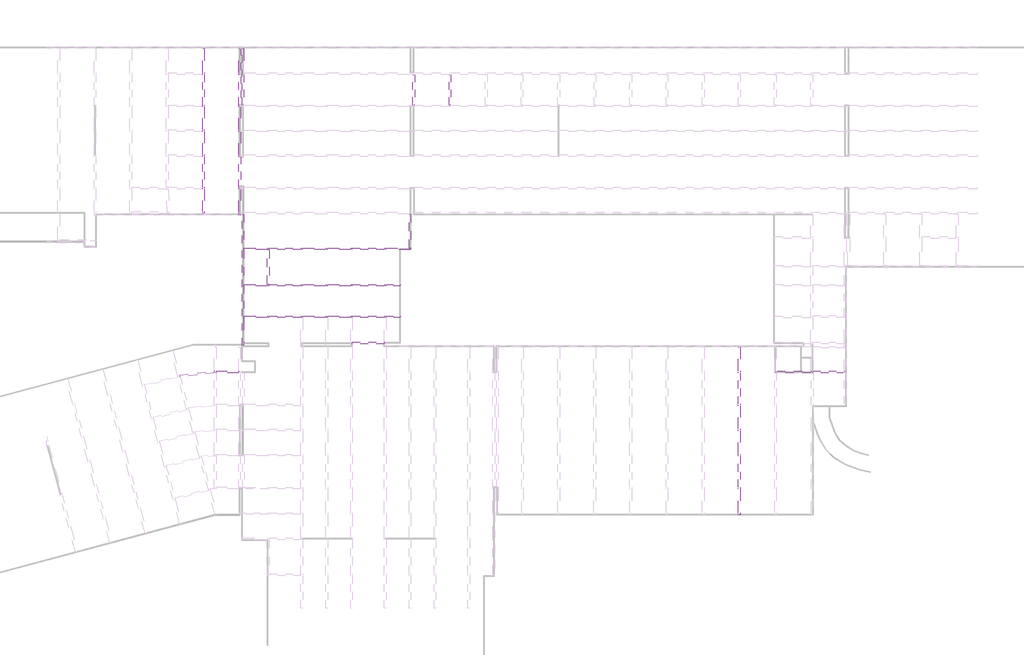
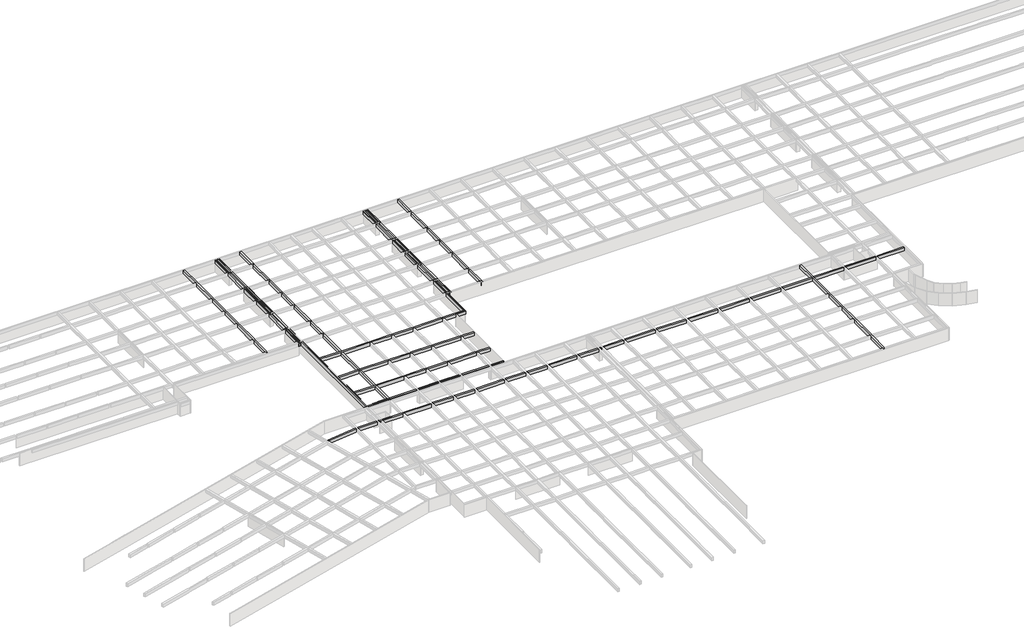
# One storey, part 10 of 14: 16 beams.
"""IFC4 building model written with IfcOpenShell, lengths in millimetres."""

from ifc_helpers import new_model, si_unit, frame, origin, place, context, project, spatial, polyline, outline, extrude, faceted_brep, element, save

model = new_model("IFC4")

# Units and contexts
model_context = context("Model", 3, world=origin())
ifc_project = project(units=[si_unit("LENGTHUNIT", "METRE", prefix="MILLI")], contexts=[model_context])

# Site, building, storey
site = spatial("IfcSite", under=ifc_project)
building = spatial("IfcBuilding", under=site)
storey = spatial("IfcBuildingStorey", under=building, Name="户型图", Elevation=0.0)

# Beams
placement = place(None, origin())
element("IfcBeam", 1, ObjectType="混凝土 - 矩形梁 : KL_beam", at=placement, inside=storey, context=model_context, shape_type="Brep", body=[
    faceted_brep([(4754.7716095, -153167.1629538, 3300.0), (5154.7716095, -153167.1629538, 3300.0), (5154.7716095, -152848.950757, 3300.0), (5154.7716095, -147899.284307, 3300.0), (5154.7716095, -147499.284307, 3300.0), (5154.7716095, -140920.0179086, 3300.0), (5154.7716095, -140520.0179086, 3300.0), (5154.7716095, -135526.4975491, 3300.0), (5154.7716095, -135126.4975491, 3300.0), (5154.7716095, -130180.0179086, 3300.0), (5154.7716095, -129780.0179086, 3300.0), (5154.7716095, -123258.950757, 3300.0), (5154.7716095, -122858.950757, 3300.0), (5154.7716095, -117558.950757, 3300.0), (4754.7716095, -117558.950757, 3300.0), (4754.7716095, -122858.950757, 3300.0), (4754.7716095, -123258.950757, 3300.0), (4754.7716095, -129780.0179086, 3300.0), (4754.7716095, -130180.0179086, 3300.0), (4754.7716095, -135126.4975491, 3300.0), (4754.7716095, -135526.4975491, 3300.0), (4754.7716095, -140520.0179086, 3300.0), (4754.7716095, -140920.0179086, 3300.0), (4754.7716095, -147499.284307, 3300.0), (4754.7716095, -147899.284307, 3300.0), (4754.7716095, -152848.950757, 3300.0), (4754.7716095, -153167.1629538, 2500.0), (4754.7716095, -117558.950757, 2500.0), (4754.7716095, -122858.950757, 2500.0), (4754.7716095, -123258.950757, 2500.0), (4754.7716095, -129780.0179086, 2500.0), (4754.7716095, -130180.0179086, 2500.0), (4754.7716095, -135126.4975491, 2500.0), (4754.7716095, -135526.4975491, 2500.0), (4754.7716095, -140520.0179086, 2500.0), (4754.7716095, -140920.0179086, 2500.0), (4754.7716095, -147499.284307, 2500.0), (4754.7716095, -147899.284307, 2500.0), (4754.7716095, -152848.950757, 2500.0), (5154.7716095, -153167.1629538, 2500.0), (5154.7716095, -117558.950757, 2500.0), (5154.7716095, -122858.950757, 2500.0), (5154.7716095, -123258.950757, 2500.0), (5154.7716095, -129780.0179086, 2500.0), (5154.7716095, -130180.0179086, 2500.0), (5154.7716095, -135126.4975491, 2500.0), (5154.7716095, -135526.4975491, 2500.0), (5154.7716095, -140520.0179086, 2500.0), (5154.7716095, -140920.0179086, 2500.0), (5154.7716095, -147499.284307, 2500.0), (5154.7716095, -147899.284307, 2500.0), (5154.7716095, -152848.950757, 2500.0)], [[[0, 1, 2, 3, 4, 5, 6, 7, 8, 9, 10, 11, 12, 13, 14, 15, 16, 17, 18, 19, 20, 21, 22, 23, 24, 25]], [[26, 0, 25, 24, 23, 22, 21, 20, 19, 18, 17, 16, 15, 14, 27, 28, 29, 30, 31, 32, 33, 34, 35, 36, 37, 38]], [[39, 26, 38, 37, 36, 35, 34, 33, 32, 31, 30, 29, 28, 27, 40, 41, 42, 43, 44, 45, 46, 47, 48, 49, 50, 51]], [[1, 39, 51, 50, 49, 48, 47, 46, 45, 44, 43, 42, 41, 40, 13, 12, 11, 10, 9, 8, 7, 6, 5, 4, 3, 2]], [[1, 0, 26, 39]], [[14, 13, 40, 27]]]),
])
element("IfcBeam", 2, ObjectType="混凝土 - 矩形梁 : KL_beam", at=placement, inside=storey, context=model_context, shape_type="Brep", body=[
    faceted_brep([(12577.2949044, -153567.1629538, 3300.0), (12977.2949044, -153567.1629538, 3300.0), (12977.2949044, -153299.284307, 3300.0), (12977.2949044, -152899.284307, 3300.0), (12977.2949044, -147899.284307, 3300.0), (12977.2949044, -147499.284307, 3300.0), (12977.2949044, -140920.0179086, 3300.0), (12977.2949044, -140520.0179086, 3300.0), (12977.2949044, -135580.0179086, 3300.0), (12977.2949044, -135180.0179086, 3300.0), (12977.2949044, -130180.0179086, 3300.0), (12977.2949044, -129780.0179086, 3300.0), (12977.2949044, -117558.950757, 3300.0), (12577.2949044, -117558.950757, 3300.0), (12577.2949044, -122858.950757, 3300.0), (12577.2949044, -123258.950757, 3300.0), (12577.2949044, -129780.0179086, 3300.0), (12577.2949044, -130180.0179086, 3300.0), (12577.2949044, -135126.4975491, 3300.0), (12577.2949044, -135526.4975491, 3300.0), (12577.2949044, -140520.0179086, 3300.0), (12577.2949044, -140920.0179086, 3300.0), (12577.2949044, -147499.284307, 3300.0), (12577.2949044, -147899.284307, 3300.0), (12577.2949044, -152848.950757, 3300.0), (12577.2949044, -153248.950757, 3300.0), (12577.2949044, -153567.1629538, 2500.0), (12577.2949044, -117558.950757, 2500.0), (12577.2949044, -122858.950757, 2500.0), (12577.2949044, -123258.950757, 2500.0), (12577.2949044, -129780.0179086, 2500.0), (12577.2949044, -130180.0179086, 2500.0), (12577.2949044, -135126.4975491, 2500.0), (12577.2949044, -135526.4975491, 2500.0), (12577.2949044, -140520.0179086, 2500.0), (12577.2949044, -140920.0179086, 2500.0), (12577.2949044, -147499.284307, 2500.0), (12577.2949044, -147899.284307, 2500.0), (12577.2949044, -152848.950757, 2500.0), (12577.2949044, -153248.950757, 2500.0), (12977.2949044, -153567.1629538, 2500.0), (12977.2949044, -117558.950757, 2500.0), (12977.2949044, -129780.0179086, 2500.0), (12977.2949044, -130180.0179086, 2500.0), (12977.2949044, -135180.0179086, 2500.0), (12977.2949044, -135580.0179086, 2500.0), (12977.2949044, -140520.0179086, 2500.0), (12977.2949044, -140920.0179086, 2500.0), (12977.2949044, -147499.284307, 2500.0), (12977.2949044, -147899.284307, 2500.0), (12977.2949044, -152899.284307, 2500.0), (12977.2949044, -153299.284307, 2500.0)], [[[0, 1, 2, 3, 4, 5, 6, 7, 8, 9, 10, 11, 12, 13, 14, 15, 16, 17, 18, 19, 20, 21, 22, 23, 24, 25]], [[26, 0, 25, 24, 23, 22, 21, 20, 19, 18, 17, 16, 15, 14, 13, 27, 28, 29, 30, 31, 32, 33, 34, 35, 36, 37, 38, 39]], [[40, 26, 39, 38, 37, 36, 35, 34, 33, 32, 31, 30, 29, 28, 27, 41, 42, 43, 44, 45, 46, 47, 48, 49, 50, 51]], [[1, 40, 51, 50, 49, 48, 47, 46, 45, 44, 43, 42, 41, 12, 11, 10, 9, 8, 7, 6, 5, 4, 3, 2]], [[1, 0, 26, 40]], [[13, 12, 41, 27]]]),
])
element("IfcBeam", 3, ObjectType="混凝土 - 矩形梁 : KL_beam", at=placement, inside=storey, context=model_context, shape_type="Brep", body=[
    faceted_brep([(49716.5330009, -161020.767119, 3300.0), (49716.5330009, -160620.767119, 3300.0), (49316.5330009, -160620.767119, 3300.0), (44331.9066405, -160620.767119, 3300.0), (43931.9066405, -160620.767119, 3300.0), (37081.5607309, -160620.767119, 3300.0), (36681.5607309, -160620.767119, 3300.0), (31751.9066405, -160620.767119, 3300.0), (31351.9066405, -160620.767119, 3300.0), (26321.5607309, -160620.767119, 3300.0), (25921.5607309, -160620.767119, 3300.0), (19160.0865653, -160620.767119, 3300.0), (18760.0865653, -160620.767119, 3300.0), (13677.2949044, -160620.767119, 3300.0), (13677.2949044, -161020.767119, 3300.0), (18760.0865653, -161020.767119, 3300.0), (19160.0865653, -161020.767119, 3300.0), (25921.5607309, -161020.767119, 3300.0), (26321.5607309, -161020.767119, 3300.0), (31351.9066405, -161020.767119, 3300.0), (31751.9066405, -161020.767119, 3300.0), (36681.5607309, -161020.767119, 3300.0), (37081.5607309, -161020.767119, 3300.0), (43931.9066405, -161020.767119, 3300.0), (44331.9066405, -161020.767119, 3300.0), (49716.5330009, -161020.767119, 2500.0), (13677.2949044, -161020.767119, 2500.0), (18760.0865653, -161020.767119, 2500.0), (19160.0865653, -161020.767119, 2500.0), (25921.5607309, -161020.767119, 2500.0), (26321.5607309, -161020.767119, 2500.0), (31351.9066405, -161020.767119, 2500.0), (31751.9066405, -161020.767119, 2500.0), (36681.5607309, -161020.767119, 2500.0), (37081.5607309, -161020.767119, 2500.0), (43931.9066405, -161020.767119, 2500.0), (44331.9066405, -161020.767119, 2500.0), (49716.5330009, -160620.767119, 2500.0), (13677.2949044, -160620.767119, 2500.0), (18760.0865653, -160620.767119, 2500.0), (19160.0865653, -160620.767119, 2500.0), (25921.5607309, -160620.767119, 2500.0), (26321.5607309, -160620.767119, 2500.0), (31351.9066405, -160620.767119, 2500.0), (31751.9066405, -160620.767119, 2500.0), (36681.5607309, -160620.767119, 2500.0), (37081.5607309, -160620.767119, 2500.0), (43931.9066405, -160620.767119, 2500.0), (44331.9066405, -160620.767119, 2500.0), (49316.5330009, -160620.767119, 2500.0)], [[[0, 1, 2, 3, 4, 5, 6, 7, 8, 9, 10, 11, 12, 13, 14, 15, 16, 17, 18, 19, 20, 21, 22, 23, 24]], [[25, 0, 24, 23, 22, 21, 20, 19, 18, 17, 16, 15, 14, 26, 27, 28, 29, 30, 31, 32, 33, 34, 35, 36]], [[37, 25, 36, 35, 34, 33, 32, 31, 30, 29, 28, 27, 26, 38, 39, 40, 41, 42, 43, 44, 45, 46, 47, 48, 49]], [[1, 37, 49, 48, 47, 46, 45, 44, 43, 42, 41, 40, 39, 38, 13, 12, 11, 10, 9, 8, 7, 6, 5, 4, 3, 2]], [[14, 13, 38, 26]], [[1, 0, 25, 37]]]),
])
element("IfcBeam", 4, ObjectType="混凝土 - 矩形梁 : KL_beam", at=placement, inside=storey, context=model_context, shape_type="Brep", body=[
    faceted_brep([(47376.4139527, -168501.0793872, 3300.0), (47376.4139527, -168901.0793872, 3300.0), (47376.4139527, -168901.0793872, 2500.0), (47376.4139527, -168501.0793872, 2500.0), (44331.9066405, -168501.0793872, 3300.0), (43931.9066405, -168501.0793872, 3300.0), (37081.5607309, -168501.0793872, 3300.0), (36681.5607309, -168501.0793872, 3300.0), (31751.9066405, -168501.0793872, 3300.0), (31351.9066405, -168501.0793872, 3300.0), (26321.5607309, -168501.0793872, 3300.0), (25921.5607309, -168501.0793872, 3300.0), (19160.0865653, -168501.0793872, 3300.0), (18760.0865653, -168501.0793872, 3300.0), (13677.2949044, -168501.0793872, 3300.0), (13677.2949044, -168901.0793872, 3300.0), (18760.0865653, -168901.0793872, 3300.0), (19160.0865653, -168901.0793872, 3300.0), (25921.5607309, -168901.0793872, 3300.0), (26321.5607309, -168901.0793872, 3300.0), (31351.9066405, -168901.0793872, 3300.0), (31751.9066405, -168901.0793872, 3300.0), (36681.5607309, -168901.0793872, 3300.0), (37081.5607309, -168901.0793872, 3300.0), (43931.9066405, -168901.0793872, 3300.0), (44331.9066405, -168901.0793872, 3300.0), (13677.2949044, -168901.0793872, 2500.0), (18760.0865653, -168901.0793872, 2500.0), (19160.0865653, -168901.0793872, 2500.0), (25921.5607309, -168901.0793872, 2500.0), (26321.5607309, -168901.0793872, 2500.0), (31351.9066405, -168901.0793872, 2500.0), (31751.9066405, -168901.0793872, 2500.0), (36681.5607309, -168901.0793872, 2500.0), (37081.5607309, -168901.0793872, 2500.0), (43931.9066405, -168901.0793872, 2500.0), (44331.9066405, -168901.0793872, 2500.0), (13677.2949044, -168501.0793872, 2500.0), (18760.0865653, -168501.0793872, 2500.0), (19160.0865653, -168501.0793872, 2500.0), (25921.5607309, -168501.0793872, 2500.0), (26321.5607309, -168501.0793872, 2500.0), (31351.9066405, -168501.0793872, 2500.0), (31751.9066405, -168501.0793872, 2500.0), (36681.5607309, -168501.0793872, 2500.0), (37081.5607309, -168501.0793872, 2500.0), (43931.9066405, -168501.0793872, 2500.0), (44331.9066405, -168501.0793872, 2500.0)], [[[0, 1, 2, 3]], [[1, 0, 4, 5, 6, 7, 8, 9, 10, 11, 12, 13, 14, 15, 16, 17, 18, 19, 20, 21, 22, 23, 24, 25]], [[2, 1, 25, 24, 23, 22, 21, 20, 19, 18, 17, 16, 15, 26, 27, 28, 29, 30, 31, 32, 33, 34, 35, 36]], [[3, 2, 36, 35, 34, 33, 32, 31, 30, 29, 28, 27, 26, 37, 38, 39, 40, 41, 42, 43, 44, 45, 46, 47]], [[0, 3, 47, 46, 45, 44, 43, 42, 41, 40, 39, 38, 37, 14, 13, 12, 11, 10, 9, 8, 7, 6, 5, 4]], [[15, 14, 37, 26]]]),
])
element("IfcBeam", 5, ObjectType="混凝土 - 矩形梁 : KL_beam", at=placement, inside=storey, context=model_context, shape_type="Brep", body=[
    faceted_brep([(47376.4139526, -175317.1358924, 3300.0), (47376.4139526, -175717.1358924, 3300.0), (47376.4139526, -175717.1358924, 2500.0), (47376.4139526, -175317.1358924, 2500.0), (44331.9066405, -175317.1358924, 3300.0), (43931.9066405, -175317.1358924, 3300.0), (37081.5607309, -175317.1358924, 3300.0), (36681.5607309, -175317.1358924, 3300.0), (31751.9066405, -175317.1358924, 3300.0), (31351.9066405, -175317.1358924, 3300.0), (26321.5607309, -175317.1358924, 3300.0), (25921.5607309, -175317.1358924, 3300.0), (19160.0865653, -175317.1358924, 3300.0), (18760.0865653, -175317.1358924, 3300.0), (13677.2949044, -175317.1358924, 3300.0), (13677.2949044, -175717.1358924, 3300.0), (18760.0865653, -175717.1358924, 3300.0), (19160.0865653, -175717.1358924, 3300.0), (25921.5607309, -175717.1358924, 3300.0), (26321.5607309, -175717.1358924, 3300.0), (31351.9066405, -175717.1358924, 3300.0), (31751.9066405, -175717.1358924, 3300.0), (36681.5607309, -175717.1358924, 3300.0), (37081.5607309, -175717.1358924, 3300.0), (43931.9066405, -175717.1358924, 3300.0), (44331.9066405, -175717.1358924, 3300.0), (13677.2949044, -175717.1358924, 2500.0), (18760.0865653, -175717.1358924, 2500.0), (19160.0865653, -175717.1358924, 2500.0), (25921.5607309, -175717.1358924, 2500.0), (26321.5607309, -175717.1358924, 2500.0), (31351.9066405, -175717.1358924, 2500.0), (31751.9066405, -175717.1358924, 2500.0), (36681.5607309, -175717.1358924, 2500.0), (37081.5607309, -175717.1358924, 2500.0), (43931.9066405, -175717.1358924, 2500.0), (44331.9066405, -175717.1358924, 2500.0), (13677.2949044, -175317.1358924, 2500.0), (18760.0865653, -175317.1358924, 2500.0), (19160.0865653, -175317.1358924, 2500.0), (25921.5607309, -175317.1358924, 2500.0), (26321.5607309, -175317.1358924, 2500.0), (31351.9066405, -175317.1358924, 2500.0), (31751.9066405, -175317.1358924, 2500.0), (36681.5607309, -175317.1358924, 2500.0), (37081.5607309, -175317.1358924, 2500.0), (43931.9066405, -175317.1358924, 2500.0), (44331.9066405, -175317.1358924, 2500.0)], [[[0, 1, 2, 3]], [[1, 0, 4, 5, 6, 7, 8, 9, 10, 11, 12, 13, 14, 15, 16, 17, 18, 19, 20, 21, 22, 23, 24, 25]], [[2, 1, 25, 24, 23, 22, 21, 20, 19, 18, 17, 16, 15, 26, 27, 28, 29, 30, 31, 32, 33, 34, 35, 36]], [[3, 2, 36, 35, 34, 33, 32, 31, 30, 29, 28, 27, 26, 37, 38, 39, 40, 41, 42, 43, 44, 45, 46, 47]], [[0, 3, 47, 46, 45, 44, 43, 42, 41, 40, 39, 38, 37, 14, 13, 12, 11, 10, 9, 8, 7, 6, 5, 4]], [[15, 14, 37, 26]]]),
])
element("IfcBeam", 6, ObjectType="混凝土 - 矩形梁 : KL_beam", at=placement, inside=storey, context=model_context, shape_type="Brep", body=[
    faceted_brep([(13277.2949044, -129780.0179086, 3300.0), (13677.2949044, -129780.0179086, 3300.0), (13677.2949044, -123197.8127788, 3300.0), (13677.2949044, -122797.8127788, 3300.0), (13677.2949044, -117558.950757, 3300.0), (13277.2949044, -117558.950757, 3300.0), (13277.2949044, -129780.0179086, 2500.0), (13277.2949044, -117558.950757, 2500.0), (13677.2949044, -129780.0179086, 2500.0), (13677.2949044, -117558.950757, 2500.0), (13677.2949044, -122797.8127788, 2500.0), (13677.2949044, -123197.8127788, 2500.0)], [[[0, 1, 2, 3, 4, 5]], [[6, 0, 5, 7]], [[8, 6, 7, 9, 10, 11]], [[1, 8, 11, 10, 9, 4, 3, 2]], [[1, 0, 6, 8]], [[5, 4, 9, 7]]]),
    faceted_brep([(13677.2949044, -152899.284307, 3300.0), (13277.2949044, -152899.284307, 3300.0), (13277.2949044, -152899.284307, 2500.0), (13677.2949044, -152899.284307, 2500.0), (13277.2949044, -147899.284307, 3300.0), (13677.2949044, -147899.284307, 3300.0), (13677.2949044, -147899.284307, 2500.0), (13277.2949044, -147899.284307, 2500.0)], [[[0, 1, 2, 3]], [[4, 5, 6, 7]], [[1, 0, 5, 4]], [[2, 1, 4, 7]], [[3, 2, 7, 6]], [[0, 3, 6, 5]]]),
    faceted_brep([(13277.2949044, -130180.0179086, 3300.0), (13677.2949044, -130180.0179086, 3300.0), (13677.2949044, -130180.0179086, 2500.0), (13277.2949044, -130180.0179086, 2500.0), (13677.2949044, -135180.0179086, 3300.0), (13277.2949044, -135180.0179086, 3300.0), (13277.2949044, -135180.0179086, 2500.0), (13677.2949044, -135180.0179086, 2500.0)], [[[0, 1, 2, 3]], [[4, 5, 6, 7]], [[1, 0, 5, 4]], [[0, 3, 6, 5]], [[3, 2, 7, 6]], [[2, 1, 4, 7]]]),
    faceted_brep([(13677.2949044, -135580.0179086, 3300.0), (13277.2949044, -135580.0179086, 3300.0), (13277.2949044, -140520.0179086, 3300.0), (13677.2949044, -140520.0179086, 3300.0), (13277.2949044, -135580.0179086, 2500.0), (13277.2949044, -140520.0179086, 2500.0), (13677.2949044, -135580.0179086, 2500.0), (13677.2949044, -140520.0179086, 2500.0)], [[[0, 1, 2, 3]], [[1, 4, 5, 2]], [[4, 6, 7, 5]], [[6, 0, 3, 7]], [[1, 0, 6, 4]], [[3, 2, 5, 7]]]),
    faceted_brep([(13277.2949044, -140920.0179086, 3300.0), (13677.2949044, -140920.0179086, 3300.0), (13677.2949044, -140920.0179086, 2500.0), (13277.2949044, -140920.0179086, 2500.0), (13677.2949044, -147499.284307, 3300.0), (13277.2949044, -147499.284307, 3300.0), (13277.2949044, -147499.284307, 2500.0), (13677.2949044, -147499.284307, 2500.0)], [[[0, 1, 2, 3]], [[4, 5, 6, 7]], [[1, 0, 5, 4]], [[0, 3, 6, 5]], [[3, 2, 7, 6]], [[2, 1, 4, 7]]]),
])
element("IfcBeam", 7, ObjectType="混凝土 - 矩形梁 : KL_beam", at=placement, inside=storey, context=model_context, shape_type="Brep", body=[
    faceted_brep([(13677.2949044, -153299.284307, 3300.0), (13277.2949044, -153299.284307, 3300.0), (13277.2949044, -181668.950757, 3300.0), (13677.2949044, -181668.950757, 3300.0), (13677.2949044, -181394.9655707, 3300.0), (13677.2949044, -180994.9655707, 3300.0), (13677.2949044, -175717.1358924, 3300.0), (13677.2949044, -175317.1358924, 3300.0), (13677.2949044, -168901.0793872, 3300.0), (13677.2949044, -168501.0793872, 3300.0), (13677.2949044, -161020.767119, 3300.0), (13677.2949044, -160620.767119, 3300.0), (13277.2949044, -153299.284307, 2500.0), (13277.2949044, -181668.950757, 2500.0), (13677.2949044, -153299.284307, 2500.0), (13677.2949044, -160620.767119, 2500.0), (13677.2949044, -161020.767119, 2500.0), (13677.2949044, -168501.0793872, 2500.0), (13677.2949044, -168901.0793872, 2500.0), (13677.2949044, -175317.1358924, 2500.0), (13677.2949044, -175717.1358924, 2500.0), (13677.2949044, -180994.9655707, 2500.0), (13677.2949044, -181394.9655707, 2500.0), (13677.2949044, -181668.950757, 2500.0)], [[[0, 1, 2, 3, 4, 5, 6, 7, 8, 9, 10, 11]], [[1, 12, 13, 2]], [[12, 14, 15, 16, 17, 18, 19, 20, 21, 22, 23, 13]], [[14, 0, 11, 10, 9, 8, 7, 6, 5, 4, 3, 23, 22, 21, 20, 19, 18, 17, 16, 15]], [[1, 0, 14, 12]], [[3, 2, 13, 23]]]),
])
element("IfcBeam", 8, ObjectType="混凝土 - 矩形梁 : KL_beam", at=placement, inside=storey, context=model_context, shape_type="Brep", body=[
    faceted_brep([(19160.0865653, -175717.1358924, 3300.0), (18760.0865653, -175717.1358924, 3300.0), (18760.0865653, -180994.9655707, 3300.0), (18760.0865653, -181394.9655707, 3300.0), (18760.0865653, -181668.950757, 3300.0), (19160.0865653, -181668.950757, 3300.0), (19160.0865653, -181394.9655707, 3300.0), (19160.0865653, -180994.9655707, 3300.0), (19160.0865653, -175717.1358924, 2500.0), (19160.0865653, -181668.950757, 2500.0), (19160.0865653, -181394.9655707, 2500.0), (19160.0865653, -180994.9655707, 2500.0), (18760.0865653, -175717.1358924, 2500.0), (18760.0865653, -181668.950757, 2500.0), (18760.0865653, -181394.9655707, 2500.0), (18760.0865653, -180994.9655707, 2500.0)], [[[0, 1, 2, 3, 4, 5, 6, 7]], [[8, 0, 7, 6, 5, 9, 10, 11]], [[12, 8, 11, 10, 9, 13, 14, 15]], [[1, 12, 15, 14, 13, 4, 3, 2]], [[1, 0, 8, 12]], [[5, 4, 13, 9]]]),
    faceted_brep([(18760.0865653, -123197.8127788, 3300.0), (19160.0865653, -123197.8127788, 3300.0), (19160.0865653, -123197.8127788, 2500.0), (18760.0865653, -123197.8127788, 2500.0), (19160.0865653, -129780.0179086, 3300.0), (18760.0865653, -129780.0179086, 3300.0), (18760.0865653, -129780.0179086, 2500.0), (19160.0865653, -129780.0179086, 2500.0)], [[[0, 1, 2, 3]], [[4, 5, 6, 7]], [[1, 0, 5, 4]], [[2, 1, 4, 7]], [[3, 2, 7, 6]], [[0, 3, 6, 5]]]),
    faceted_brep([(19160.0865653, -122797.8127788, 3300.0), (18760.0865653, -122797.8127788, 3300.0), (18760.0865653, -122797.8127788, 2500.0), (19160.0865653, -122797.8127788, 2500.0), (19160.0865653, -117558.950757, 3300.0), (18760.0865653, -117558.950757, 3300.0), (19160.0865653, -117558.950757, 2500.0), (18760.0865653, -117558.950757, 2500.0)], [[[0, 1, 2, 3]], [[1, 0, 4, 5]], [[0, 3, 6, 4]], [[3, 2, 7, 6]], [[2, 1, 5, 7]], [[5, 4, 6, 7]]]),
    faceted_brep([(18760.0865653, -130180.0179086, 3300.0), (19160.0865653, -130180.0179086, 3300.0), (19160.0865653, -130180.0179086, 2500.0), (18760.0865653, -130180.0179086, 2500.0), (19160.0865653, -135180.0179086, 3300.0), (18760.0865653, -135180.0179086, 3300.0), (18760.0865653, -135180.0179086, 2500.0), (19160.0865653, -135180.0179086, 2500.0)], [[[0, 1, 2, 3]], [[4, 5, 6, 7]], [[1, 0, 5, 4]], [[2, 1, 4, 7]], [[3, 2, 7, 6]], [[0, 3, 6, 5]]]),
    faceted_brep([(18760.0865653, -135580.0179086, 3300.0), (19160.0865653, -135580.0179086, 3300.0), (19160.0865653, -135580.0179086, 2500.0), (18760.0865653, -135580.0179086, 2500.0), (19160.0865653, -140520.0179086, 3300.0), (18760.0865653, -140520.0179086, 3300.0), (18760.0865653, -140520.0179086, 2500.0), (19160.0865653, -140520.0179086, 2500.0)], [[[0, 1, 2, 3]], [[4, 5, 6, 7]], [[1, 0, 5, 4]], [[2, 1, 4, 7]], [[3, 2, 7, 6]], [[0, 3, 6, 5]]]),
    faceted_brep([(18760.0865653, -140920.0179086, 3300.0), (19160.0865653, -140920.0179086, 3300.0), (19160.0865653, -140920.0179086, 2500.0), (18760.0865653, -140920.0179086, 2500.0), (19160.0865653, -147499.284307, 3300.0), (18760.0865653, -147499.284307, 3300.0), (18760.0865653, -147499.284307, 2500.0), (19160.0865653, -147499.284307, 2500.0)], [[[0, 1, 2, 3]], [[4, 5, 6, 7]], [[1, 0, 5, 4]], [[2, 1, 4, 7]], [[3, 2, 7, 6]], [[0, 3, 6, 5]]]),
    faceted_brep([(18760.0865653, -147899.284307, 3300.0), (19160.0865653, -147899.284307, 3300.0), (19160.0865653, -147899.284307, 2500.0), (18760.0865653, -147899.284307, 2500.0), (19160.0865653, -152899.284307, 3300.0), (18760.0865653, -152899.284307, 3300.0), (18760.0865653, -152899.284307, 2500.0), (19160.0865653, -152899.284307, 2500.0)], [[[0, 1, 2, 3]], [[4, 5, 6, 7]], [[1, 0, 5, 4]], [[2, 1, 4, 7]], [[3, 2, 7, 6]], [[0, 3, 6, 5]]]),
    faceted_brep([(18760.0865653, -153299.284307, 3300.0), (19160.0865653, -153299.284307, 3300.0), (19160.0865653, -153299.284307, 2500.0), (18760.0865653, -153299.284307, 2500.0), (19160.0865653, -160620.767119, 3300.0), (18760.0865653, -160620.767119, 3300.0), (18760.0865653, -160620.767119, 2500.0), (19160.0865653, -160620.767119, 2500.0)], [[[0, 1, 2, 3]], [[4, 5, 6, 7]], [[1, 0, 5, 4]], [[2, 1, 4, 7]], [[3, 2, 7, 6]], [[0, 3, 6, 5]]]),
    faceted_brep([(18760.0865653, -161020.767119, 3300.0), (19160.0865653, -161020.767119, 3300.0), (19160.0865653, -161020.767119, 2500.0), (18760.0865653, -161020.767119, 2500.0), (19160.0865653, -168501.0793872, 3300.0), (18760.0865653, -168501.0793872, 3300.0), (18760.0865653, -168501.0793872, 2500.0), (19160.0865653, -168501.0793872, 2500.0)], [[[0, 1, 2, 3]], [[4, 5, 6, 7]], [[1, 0, 5, 4]], [[2, 1, 4, 7]], [[3, 2, 7, 6]], [[0, 3, 6, 5]]]),
    faceted_brep([(18760.0865653, -168901.0793872, 3300.0), (19160.0865653, -168901.0793872, 3300.0), (19160.0865653, -168901.0793872, 2500.0), (18760.0865653, -168901.0793872, 2500.0), (19160.0865653, -175317.1358924, 3300.0), (18760.0865653, -175317.1358924, 3300.0), (18760.0865653, -175317.1358924, 2500.0), (19160.0865653, -175317.1358924, 2500.0)], [[[0, 1, 2, 3]], [[4, 5, 6, 7]], [[1, 0, 5, 4]], [[2, 1, 4, 7]], [[3, 2, 7, 6]], [[0, 3, 6, 5]]]),
])
element("IfcBeam", 9, ObjectType="混凝土 - 矩形梁 : KL_beam", at=placement, inside=storey, context=model_context, shape_type="SweptSolid", body=[
    extrude(outline(polyline([(49716.5330009, -122797.8127788), (49316.5330009, -122797.8127788), (49316.5330009, -117558.950757), (49716.5330009, -117558.950757), (49716.5330009, -122797.8127788)])), frame((0.0, 0.0, 2500.0), z_axis=(0.0, 0.0, 1.0), x_axis=(1.0, 0.0, 0.0)), (0.0, 0.0, 1.0), 800.0),
    extrude(outline(polyline([(49716.5330009, -160620.767119), (49316.5330009, -160620.767119), (49316.5330009, -153299.284307), (49716.5330009, -153299.284307), (49716.5330009, -160620.767119)])), frame((0.0, 0.0, 2500.0), z_axis=(0.0, 0.0, 1.0), x_axis=(1.0, 0.0, 0.0)), (0.0, 0.0, 1.0), 800.0),
    extrude(outline(polyline([(49316.5330009, -123197.8127788), (49716.5330009, -123197.8127788), (49716.5330009, -129780.0179086), (49316.5330009, -129780.0179086), (49316.5330009, -123197.8127788)])), frame((0.0, 0.0, 2500.0), z_axis=(0.0, 0.0, 1.0), x_axis=(1.0, 0.0, 0.0)), (0.0, 0.0, 1.0), 800.0),
    extrude(outline(polyline([(49316.5330009, -130180.0179086), (49716.5330009, -130180.0179086), (49716.5330009, -135180.0179086), (49316.5330009, -135180.0179086), (49316.5330009, -130180.0179086)])), frame((0.0, 0.0, 2500.0), z_axis=(0.0, 0.0, 1.0), x_axis=(1.0, 0.0, 0.0)), (0.0, 0.0, 1.0), 800.0),
    extrude(outline(polyline([(49316.5330009, -135580.0179086), (49716.5330009, -135580.0179086), (49716.5330009, -140520.0179086), (49316.5330009, -140520.0179086), (49316.5330009, -135580.0179086)])), frame((0.0, 0.0, 2500.0), z_axis=(0.0, 0.0, 1.0), x_axis=(1.0, 0.0, 0.0)), (0.0, 0.0, 1.0), 800.0),
    extrude(outline(polyline([(49316.5330009, -140920.0179086), (49716.5330009, -140920.0179086), (49716.5330009, -147499.284307), (49316.5330009, -147499.284307), (49316.5330009, -140920.0179086)])), frame((0.0, 0.0, 2500.0), z_axis=(0.0, 0.0, 1.0), x_axis=(1.0, 0.0, 0.0)), (0.0, 0.0, 1.0), 800.0),
    extrude(outline(polyline([(49316.5330009, -147899.284307), (49716.5330009, -147899.284307), (49716.5330009, -152899.284307), (49316.5330009, -152899.284307), (49316.5330009, -147899.284307)])), frame((0.0, 0.0, 2500.0), z_axis=(0.0, 0.0, 1.0), x_axis=(1.0, 0.0, 0.0)), (0.0, 0.0, 1.0), 800.0),
])
element("IfcBeam", 10, ObjectType="混凝土 - 矩形梁 : KL_beam", at=placement, inside=storey, context=model_context, shape_type="SweptSolid", body=[
    extrude(outline(polyline([(50537.2949044, -153358.950757), (50137.2949044, -153358.950757), (50137.2949044, -153299.284307), (50537.2949044, -153299.284307), (50537.2949044, -153358.950757)])), frame((0.0, 0.0, 2500.0), z_axis=(0.0, 0.0, 1.0), x_axis=(1.0, 0.0, 0.0)), (0.0, 0.0, 1.0), 800.0),
    extrude(outline(polyline([(50137.2949044, -123197.8127788), (50537.2949044, -123197.8127788), (50537.2949044, -129780.0179086), (50137.2949044, -129780.0179086), (50137.2949044, -123197.8127788)])), frame((0.0, 0.0, 2500.0), z_axis=(0.0, 0.0, 1.0), x_axis=(1.0, 0.0, 0.0)), (0.0, 0.0, 1.0), 800.0),
    extrude(outline(polyline([(50537.2949044, -122797.8127788), (50137.2949044, -122797.8127788), (50137.2949044, -117558.950757), (50537.2949044, -117558.950757), (50537.2949044, -122797.8127788)])), frame((0.0, 0.0, 2500.0), z_axis=(0.0, 0.0, 1.0), x_axis=(1.0, 0.0, 0.0)), (0.0, 0.0, 1.0), 800.0),
    extrude(outline(polyline([(50137.2949044, -130180.0179086), (50537.2949044, -130180.0179086), (50537.2949044, -135180.0179086), (50137.2949044, -135180.0179086), (50137.2949044, -130180.0179086)])), frame((0.0, 0.0, 2500.0), z_axis=(0.0, 0.0, 1.0), x_axis=(1.0, 0.0, 0.0)), (0.0, 0.0, 1.0), 800.0),
    extrude(outline(polyline([(50137.2949044, -135580.0179086), (50537.2949044, -135580.0179086), (50537.2949044, -140520.0179086), (50137.2949044, -140520.0179086), (50137.2949044, -135580.0179086)])), frame((0.0, 0.0, 2500.0), z_axis=(0.0, 0.0, 1.0), x_axis=(1.0, 0.0, 0.0)), (0.0, 0.0, 1.0), 800.0),
    extrude(outline(polyline([(50137.2949044, -140920.0179086), (50537.2949044, -140920.0179086), (50537.2949044, -147499.284307), (50137.2949044, -147499.284307), (50137.2949044, -140920.0179086)])), frame((0.0, 0.0, 2500.0), z_axis=(0.0, 0.0, 1.0), x_axis=(1.0, 0.0, 0.0)), (0.0, 0.0, 1.0), 800.0),
    extrude(outline(polyline([(50137.2949044, -147899.284307), (50537.2949044, -147899.284307), (50537.2949044, -152899.284307), (50137.2949044, -152899.284307), (50137.2949044, -147899.284307)])), frame((0.0, 0.0, 2500.0), z_axis=(0.0, 0.0, 1.0), x_axis=(1.0, 0.0, 0.0)), (0.0, 0.0, 1.0), 800.0),
])
element("IfcBeam", 11, ObjectType="混凝土 - 矩形梁 : KL_beam", at=placement, inside=storey, context=model_context, shape_type="SweptSolid", body=[
    extrude(outline(polyline([(58330.1134745, -153358.950757), (57930.1134745, -153358.950757), (57930.1134745, -153299.284307), (58330.1134745, -153299.284307), (58330.1134745, -153358.950757)])), frame((0.0, 0.0, 2500.0), z_axis=(0.0, 0.0, 1.0), x_axis=(1.0, 0.0, 0.0)), (0.0, 0.0, 1.0), 800.0),
    extrude(outline(polyline([(58330.1134745, -122797.8127788), (57930.1134745, -122797.8127788), (57930.1134745, -117558.950757), (58330.1134745, -117558.950757), (58330.1134745, -122797.8127788)])), frame((0.0, 0.0, 2500.0), z_axis=(0.0, 0.0, 1.0), x_axis=(1.0, 0.0, 0.0)), (0.0, 0.0, 1.0), 800.0),
    extrude(outline(polyline([(57930.1134745, -123197.8127788), (58330.1134745, -123197.8127788), (58330.1134745, -129780.0179086), (57930.1134745, -129780.0179086), (57930.1134745, -123197.8127788)])), frame((0.0, 0.0, 2500.0), z_axis=(0.0, 0.0, 1.0), x_axis=(1.0, 0.0, 0.0)), (0.0, 0.0, 1.0), 800.0),
    extrude(outline(polyline([(57930.1134745, -130180.0179086), (58330.1134745, -130180.0179086), (58330.1134745, -135180.0179086), (57930.1134745, -135180.0179086), (57930.1134745, -130180.0179086)])), frame((0.0, 0.0, 2500.0), z_axis=(0.0, 0.0, 1.0), x_axis=(1.0, 0.0, 0.0)), (0.0, 0.0, 1.0), 800.0),
    extrude(outline(polyline([(57930.1134745, -135580.0179086), (58330.1134745, -135580.0179086), (58330.1134745, -140520.0179086), (57930.1134745, -140520.0179086), (57930.1134745, -135580.0179086)])), frame((0.0, 0.0, 2500.0), z_axis=(0.0, 0.0, 1.0), x_axis=(1.0, 0.0, 0.0)), (0.0, 0.0, 1.0), 800.0),
    extrude(outline(polyline([(57930.1134745, -140920.0179086), (58330.1134745, -140920.0179086), (58330.1134745, -147499.284307), (57930.1134745, -147499.284307), (57930.1134745, -140920.0179086)])), frame((0.0, 0.0, 2500.0), z_axis=(0.0, 0.0, 1.0), x_axis=(1.0, 0.0, 0.0)), (0.0, 0.0, 1.0), 800.0),
    extrude(outline(polyline([(57930.1134745, -147899.284307), (58330.1134745, -147899.284307), (58330.1134745, -152899.284307), (57930.1134745, -152899.284307), (57930.1134745, -147899.284307)])), frame((0.0, 0.0, 2500.0), z_axis=(0.0, 0.0, 1.0), x_axis=(1.0, 0.0, 0.0)), (0.0, 0.0, 1.0), 800.0),
])
element("IfcBeam", 12, ObjectType="混凝土 - 矩形梁 : KL_beam", at=placement, inside=storey, context=model_context, shape_type="SweptSolid", body=[
    extrude(outline(polyline([(47376.4139526, -180994.9655707), (47376.4139526, -181394.9655707), (44331.9066405, -181394.9655707), (44331.9066405, -180994.9655707), (47376.4139526, -180994.9655707)])), frame((0.0, 0.0, 2500.0), z_axis=(0.0, 0.0, 1.0), x_axis=(1.0, 0.0, 0.0)), (0.0, 0.0, 1.0), 800.0),
    extrude(outline(polyline([(13677.2949044, -181394.9655707), (13677.2949044, -180994.9655707), (18760.0865653, -180994.9655707), (18760.0865653, -181394.9655707), (13677.2949044, -181394.9655707)])), frame((0.0, 0.0, 2500.0), z_axis=(0.0, 0.0, 1.0), x_axis=(1.0, 0.0, 0.0)), (0.0, 0.0, 1.0), 800.0),
    extrude(outline(polyline([(19160.0865653, -181394.9655707), (19160.0865653, -180994.9655707), (25921.5607309, -180994.9655707), (25921.5607309, -181394.9655707), (19160.0865653, -181394.9655707)])), frame((0.0, 0.0, 2500.0), z_axis=(0.0, 0.0, 1.0), x_axis=(1.0, 0.0, 0.0)), (0.0, 0.0, 1.0), 800.0),
    extrude(outline(polyline([(26321.5607309, -181394.9655707), (26321.5607309, -180994.9655707), (31351.9066405, -180994.9655707), (31351.9066405, -181394.9655707), (26321.5607309, -181394.9655707)])), frame((0.0, 0.0, 2500.0), z_axis=(0.0, 0.0, 1.0), x_axis=(1.0, 0.0, 0.0)), (0.0, 0.0, 1.0), 800.0),
    extrude(outline(polyline([(31751.9066405, -181394.9655707), (31751.9066405, -180994.9655707), (36681.5607309, -180994.9655707), (36681.5607309, -181394.9655707), (31751.9066405, -181394.9655707)])), frame((0.0, 0.0, 2500.0), z_axis=(0.0, 0.0, 1.0), x_axis=(1.0, 0.0, 0.0)), (0.0, 0.0, 1.0), 800.0),
    extrude(outline(polyline([(37081.5607309, -181394.9655707), (37081.5607309, -180994.9655707), (43931.9066405, -180994.9655707), (43931.9066405, -181394.9655707), (37081.5607309, -181394.9655707)])), frame((0.0, 0.0, 2500.0), z_axis=(0.0, 0.0, 1.0), x_axis=(1.0, 0.0, 0.0)), (0.0, 0.0, 1.0), 800.0),
])
element("IfcBeam", 13, ObjectType="混凝土 - 矩形梁 : KL_beam", at=placement, inside=storey, context=model_context, shape_type="Brep", body=[
    faceted_brep([(120767.2949044, -218258.950757, 3300.0), (120367.2949044, -218258.950757, 3300.0), (120367.2949044, -218258.950757, 2500.0), (120767.2949044, -218258.950757, 2500.0), (120767.2949044, -218208.950757, 3300.0), (120767.2949044, -217808.950757, 3300.0), (120767.2949044, -212708.950757, 3300.0), (120767.2949044, -212308.950757, 3300.0), (120767.2949044, -205576.1028577, 3300.0), (120767.2949044, -205176.1028577, 3300.0), (120767.2949044, -200154.952508, 3300.0), (120767.2949044, -199754.952508, 3300.0), (120767.2949044, -194741.3993539, 3300.0), (120767.2949044, -194341.3993539, 3300.0), (120767.2949044, -187598.950757, 3300.0), (120767.2949044, -187198.950757, 3300.0), (120767.2949044, -182068.950757, 3300.0), (120367.2949044, -182068.950757, 3300.0), (120367.2949044, -187198.950757, 3300.0), (120367.2949044, -187598.950757, 3300.0), (120367.2949044, -194341.3993539, 3300.0), (120367.2949044, -194741.3993539, 3300.0), (120367.2949044, -199754.952508, 3300.0), (120367.2949044, -200154.952508, 3300.0), (120367.2949044, -205176.1028577, 3300.0), (120367.2949044, -205576.1028577, 3300.0), (120367.2949044, -212308.950757, 3300.0), (120367.2949044, -212708.950757, 3300.0), (120367.2949044, -217808.950757, 3300.0), (120367.2949044, -218208.950757, 3300.0), (120367.2949044, -182068.950757, 2500.0), (120367.2949044, -187198.950757, 2500.0), (120367.2949044, -187598.950757, 2500.0), (120367.2949044, -194341.3993539, 2500.0), (120367.2949044, -194741.3993539, 2500.0), (120367.2949044, -199754.952508, 2500.0), (120367.2949044, -200154.952508, 2500.0), (120367.2949044, -205176.1028577, 2500.0), (120367.2949044, -205576.1028577, 2500.0), (120367.2949044, -212308.950757, 2500.0), (120367.2949044, -212708.950757, 2500.0), (120367.2949044, -217808.950757, 2500.0), (120367.2949044, -218208.950757, 2500.0), (120767.2949044, -182068.950757, 2500.0), (120767.2949044, -187198.950757, 2500.0), (120767.2949044, -187598.950757, 2500.0), (120767.2949044, -194341.3993539, 2500.0), (120767.2949044, -194741.3993539, 2500.0), (120767.2949044, -199754.952508, 2500.0), (120767.2949044, -200154.952508, 2500.0), (120767.2949044, -205176.1028577, 2500.0), (120767.2949044, -205576.1028577, 2500.0), (120767.2949044, -212308.950757, 2500.0), (120767.2949044, -212708.950757, 2500.0), (120767.2949044, -217808.950757, 2500.0), (120767.2949044, -218208.950757, 2500.0)], [[[0, 1, 2, 3]], [[1, 0, 4, 5, 6, 7, 8, 9, 10, 11, 12, 13, 14, 15, 16, 17, 18, 19, 20, 21, 22, 23, 24, 25, 26, 27, 28, 29]], [[2, 1, 29, 28, 27, 26, 25, 24, 23, 22, 21, 20, 19, 18, 17, 30, 31, 32, 33, 34, 35, 36, 37, 38, 39, 40, 41, 42]], [[3, 2, 42, 41, 40, 39, 38, 37, 36, 35, 34, 33, 32, 31, 30, 43, 44, 45, 46, 47, 48, 49, 50, 51, 52, 53, 54, 55]], [[0, 3, 55, 54, 53, 52, 51, 50, 49, 48, 47, 46, 45, 44, 43, 16, 15, 14, 13, 12, 11, 10, 9, 8, 7, 6, 5, 4]], [[17, 16, 43, 30]]]),
])
element("IfcBeam", 14, ObjectType="混凝土 - 矩形梁 : KL_beam", at=placement, inside=storey, context=model_context, shape_type="Brep", body=[
    faceted_brep([(128549.172254, -187198.950757, 3300.0), (128549.172254, -187598.950757, 3300.0), (136047.2949044, -187598.950757, 3300.0), (136447.2949044, -187598.950757, 3300.0), (143227.2949044, -187598.950757, 3300.0), (143227.2949044, -187198.950757, 3300.0), (136347.2949044, -187198.950757, 3300.0), (135947.2949044, -187198.950757, 3300.0), (128549.172254, -187198.950757, 2500.0), (143227.2949044, -187198.950757, 2500.0), (136347.2949044, -187198.950757, 2500.0), (135947.2949044, -187198.950757, 2500.0), (128549.172254, -187598.950757, 2500.0), (143227.2949044, -187598.950757, 2500.0), (136447.2949044, -187598.950757, 2500.0), (136047.2949044, -187598.950757, 2500.0)], [[[0, 1, 2, 3, 4, 5, 6, 7]], [[8, 0, 7, 6, 5, 9, 10, 11]], [[12, 8, 11, 10, 9, 13, 14, 15]], [[1, 12, 15, 14, 13, 4, 3, 2]], [[1, 0, 8, 12]], [[5, 4, 13, 9]]]),
    faceted_brep([(25921.5607309, -187198.950757, 3300.0), (25921.5607309, -187598.950757, 3300.0), (25921.5607309, -187598.950757, 2500.0), (25921.5607309, -187198.950757, 2500.0), (19160.0865653, -187198.950757, 3300.0), (18760.0865653, -187198.950757, 3300.0), (13777.4621399, -187198.950757, 3300.0), (13377.4621399, -187198.950757, 3300.0), (12933.1378826, -187198.950757, 3300.0), (12933.1378826, -187598.950757, 3300.0), (13377.4621399, -187598.950757, 3300.0), (13777.4621399, -187598.950757, 3300.0), (18760.0865653, -187598.950757, 3300.0), (19160.0865653, -187598.950757, 3300.0), (19160.0865653, -187198.950757, 2500.0), (18760.0865653, -187198.950757, 2500.0), (13777.4621399, -187198.950757, 2500.0), (13377.4621399, -187198.950757, 2500.0), (12933.1378826, -187198.950757, 2500.0), (19160.0865653, -187598.950757, 2500.0), (18760.0865653, -187598.950757, 2500.0), (13777.4621399, -187598.950757, 2500.0), (13377.4621399, -187598.950757, 2500.0), (12933.1378826, -187598.950757, 2500.0)], [[[0, 1, 2, 3]], [[1, 0, 4, 5, 6, 7, 8, 9, 10, 11, 12, 13]], [[0, 3, 14, 15, 16, 17, 18, 8, 7, 6, 5, 4]], [[3, 2, 19, 20, 21, 22, 23, 18, 17, 16, 15, 14]], [[2, 1, 13, 12, 11, 10, 9, 23, 22, 21, 20, 19]], [[9, 8, 18, 23]]]),
    faceted_brep([(26321.5607309, -187598.950757, 3300.0), (26321.5607309, -187198.950757, 3300.0), (26321.5607309, -187198.950757, 2500.0), (26321.5607309, -187598.950757, 2500.0), (31351.9066405, -187198.950757, 3300.0), (31351.9066405, -187598.950757, 3300.0), (31351.9066405, -187598.950757, 2500.0), (31351.9066405, -187198.950757, 2500.0)], [[[0, 1, 2, 3]], [[4, 5, 6, 7]], [[1, 0, 5, 4]], [[2, 1, 4, 7]], [[3, 2, 7, 6]], [[0, 3, 6, 5]]]),
    faceted_brep([(31751.9066405, -187598.950757, 3300.0), (31751.9066405, -187198.950757, 3300.0), (31751.9066405, -187198.950757, 2500.0), (31751.9066405, -187598.950757, 2500.0), (36681.5607309, -187198.950757, 3300.0), (36681.5607309, -187598.950757, 3300.0), (36681.5607309, -187598.950757, 2500.0), (36681.5607309, -187198.950757, 2500.0)], [[[0, 1, 2, 3]], [[4, 5, 6, 7]], [[1, 0, 5, 4]], [[2, 1, 4, 7]], [[3, 2, 7, 6]], [[0, 3, 6, 5]]]),
    faceted_brep([(37081.5607309, -187598.950757, 3300.0), (37081.5607309, -187198.950757, 3300.0), (37081.5607309, -187198.950757, 2500.0), (37081.5607309, -187598.950757, 2500.0), (43931.9066405, -187198.950757, 3300.0), (43931.9066405, -187598.950757, 3300.0), (43931.9066405, -187598.950757, 2500.0), (43931.9066405, -187198.950757, 2500.0)], [[[0, 1, 2, 3]], [[4, 5, 6, 7]], [[1, 0, 5, 4]], [[2, 1, 4, 7]], [[3, 2, 7, 6]], [[0, 3, 6, 5]]]),
    faceted_brep([(44331.9066405, -187598.950757, 3300.0), (44331.9066405, -187198.950757, 3300.0), (44331.9066405, -187198.950757, 2500.0), (44331.9066405, -187598.950757, 2500.0), (49289.9831968, -187198.950757, 3300.0), (49289.9831968, -187598.950757, 3300.0), (49289.9831968, -187598.950757, 2500.0), (49289.9831968, -187198.950757, 2500.0)], [[[0, 1, 2, 3]], [[4, 5, 6, 7]], [[1, 0, 5, 4]], [[2, 1, 4, 7]], [[3, 2, 7, 6]], [[0, 3, 6, 5]]]),
    faceted_brep([(49689.9831968, -187598.950757, 3300.0), (49689.9831968, -187198.950757, 3300.0), (49689.9831968, -187198.950757, 2500.0), (49689.9831968, -187598.950757, 2500.0), (54689.9831968, -187198.950757, 3300.0), (54689.9831968, -187598.950757, 3300.0), (54689.9831968, -187598.950757, 2500.0), (54689.9831968, -187198.950757, 2500.0)], [[[0, 1, 2, 3]], [[4, 5, 6, 7]], [[1, 0, 5, 4]], [[2, 1, 4, 7]], [[3, 2, 7, 6]], [[0, 3, 6, 5]]]),
    faceted_brep([(55089.9831968, -187598.950757, 3300.0), (55089.9831968, -187198.950757, 3300.0), (55089.9831968, -187198.950757, 2500.0), (55089.9831968, -187598.950757, 2500.0), (61967.2949044, -187198.950757, 3300.0), (61967.2949044, -187598.950757, 3300.0), (61967.2949044, -187598.950757, 2500.0), (61967.2949044, -187198.950757, 2500.0)], [[[0, 1, 2, 3]], [[4, 5, 6, 7]], [[1, 0, 5, 4]], [[2, 1, 4, 7]], [[3, 2, 7, 6]], [[0, 3, 6, 5]]]),
    faceted_brep([(62367.2949044, -187598.950757, 3300.0), (62367.2949044, -187198.950757, 3300.0), (62367.2949044, -187198.950757, 2500.0), (62367.2949044, -187598.950757, 2500.0), (67367.2949044, -187198.950757, 3300.0), (67367.2949044, -187598.950757, 3300.0), (67367.2949044, -187598.950757, 2500.0), (67367.2949044, -187198.950757, 2500.0)], [[[0, 1, 2, 3]], [[4, 5, 6, 7]], [[1, 0, 5, 4]], [[2, 1, 4, 7]], [[3, 2, 7, 6]], [[0, 3, 6, 5]]]),
    faceted_brep([(67767.2949044, -187598.950757, 3300.0), (67767.2949044, -187198.950757, 3300.0), (67767.2949044, -187198.950757, 2500.0), (67767.2949044, -187598.950757, 2500.0), (68177.2949044, -187198.950757, 3300.0), (68177.2949044, -187598.950757, 3300.0), (68177.2949044, -187598.950757, 2500.0), (68177.2949044, -187198.950757, 2500.0)], [[[0, 1, 2, 3]], [[4, 5, 6, 7]], [[1, 0, 5, 4]], [[2, 1, 4, 7]], [[3, 2, 7, 6]], [[0, 3, 6, 5]]]),
    faceted_brep([(68577.2949044, -187598.950757, 3300.0), (68577.2949044, -187198.950757, 3300.0), (68577.2949044, -187198.950757, 2500.0), (68577.2949044, -187598.950757, 2500.0), (73579.8514216, -187198.950757, 3300.0), (73579.8514216, -187598.950757, 3300.0), (73579.8514216, -187598.950757, 2500.0), (73579.8514216, -187198.950757, 2500.0)], [[[0, 1, 2, 3]], [[4, 5, 6, 7]], [[1, 0, 5, 4]], [[2, 1, 4, 7]], [[3, 2, 7, 6]], [[0, 3, 6, 5]]]),
    faceted_brep([(73979.8514216, -187598.950757, 3300.0), (73979.8514216, -187198.950757, 3300.0), (73979.8514216, -187198.950757, 2500.0), (73979.8514216, -187598.950757, 2500.0), (81379.8514216, -187198.950757, 3300.0), (81379.8514216, -187598.950757, 3300.0), (81379.8514216, -187598.950757, 2500.0), (81379.8514216, -187198.950757, 2500.0)], [[[0, 1, 2, 3]], [[4, 5, 6, 7]], [[1, 0, 5, 4]], [[2, 1, 4, 7]], [[3, 2, 7, 6]], [[0, 3, 6, 5]]]),
    faceted_brep([(81779.8514216, -187598.950757, 3300.0), (81779.8514216, -187198.950757, 3300.0), (81779.8514216, -187198.950757, 2500.0), (81779.8514216, -187598.950757, 2500.0), (89134.3329203, -187198.950757, 3300.0), (89134.3329203, -187598.950757, 3300.0), (89134.3329203, -187598.950757, 2500.0), (89134.3329203, -187198.950757, 2500.0)], [[[0, 1, 2, 3]], [[4, 5, 6, 7]], [[1, 0, 5, 4]], [[2, 1, 4, 7]], [[3, 2, 7, 6]], [[0, 3, 6, 5]]]),
    faceted_brep([(89534.3329203, -187598.950757, 3300.0), (89534.3329203, -187198.950757, 3300.0), (89534.3329203, -187198.950757, 2500.0), (89534.3329203, -187598.950757, 2500.0), (96934.3329203, -187198.950757, 3300.0), (96934.3329203, -187598.950757, 3300.0), (96934.3329203, -187598.950757, 2500.0), (96934.3329203, -187198.950757, 2500.0)], [[[0, 1, 2, 3]], [[4, 5, 6, 7]], [[1, 0, 5, 4]], [[2, 1, 4, 7]], [[3, 2, 7, 6]], [[0, 3, 6, 5]]]),
    faceted_brep([(97334.3329203, -187598.950757, 3300.0), (97334.3329203, -187198.950757, 3300.0), (97334.3329203, -187198.950757, 2500.0), (97334.3329203, -187598.950757, 2500.0), (104734.3329203, -187198.950757, 3300.0), (104734.3329203, -187598.950757, 3300.0), (104734.3329203, -187598.950757, 2500.0), (104734.3329203, -187198.950757, 2500.0)], [[[0, 1, 2, 3]], [[4, 5, 6, 7]], [[1, 0, 5, 4]], [[2, 1, 4, 7]], [[3, 2, 7, 6]], [[0, 3, 6, 5]]]),
    faceted_brep([(105134.3329203, -187598.950757, 3300.0), (105134.3329203, -187198.950757, 3300.0), (105134.3329203, -187198.950757, 2500.0), (105134.3329203, -187598.950757, 2500.0), (112555.6695954, -187198.950757, 3300.0), (112555.6695954, -187598.950757, 3300.0), (112555.6695954, -187598.950757, 2500.0), (112555.6695954, -187198.950757, 2500.0)], [[[0, 1, 2, 3]], [[4, 5, 6, 7]], [[1, 0, 5, 4]], [[2, 1, 4, 7]], [[3, 2, 7, 6]], [[0, 3, 6, 5]]]),
    faceted_brep([(112955.6695954, -187598.950757, 3300.0), (112955.6695954, -187198.950757, 3300.0), (112955.6695954, -187198.950757, 2500.0), (112955.6695954, -187598.950757, 2500.0), (120367.2949044, -187198.950757, 3300.0), (120367.2949044, -187598.950757, 3300.0), (120367.2949044, -187598.950757, 2500.0), (120367.2949044, -187198.950757, 2500.0)], [[[0, 1, 2, 3]], [[4, 5, 6, 7]], [[1, 0, 5, 4]], [[2, 1, 4, 7]], [[3, 2, 7, 6]], [[0, 3, 6, 5]]]),
    faceted_brep([(120767.2949044, -187598.950757, 3300.0), (120767.2949044, -187198.950757, 3300.0), (120767.2949044, -187198.950757, 2500.0), (120767.2949044, -187598.950757, 2500.0), (128149.172254, -187198.950757, 3300.0), (128149.172254, -187598.950757, 3300.0), (128149.172254, -187598.950757, 2500.0), (128149.172254, -187198.950757, 2500.0)], [[[0, 1, 2, 3]], [[4, 5, 6, 7]], [[1, 0, 5, 4]], [[2, 1, 4, 7]], [[3, 2, 7, 6]], [[0, 3, 6, 5]]]),
])
element("IfcBeam", 15, ObjectType="混凝土 - 矩形梁 : KL_beam", at=placement, inside=storey, context=model_context, shape_type="SweptSolid", body=[
    extrude(outline(polyline([(-111.6428577, -188503.9319111), (-216.2530139, -188113.5214934), (7322.5700952, -187221.2267128), (7322.5700952, -187624.0187841), (-111.6428577, -188503.9319111)])), frame((0.0, 0.0, 2500.0), z_axis=(0.0, 0.0, 1.0), x_axis=(1.0, 0.0, 0.0)), (0.0, 0.0, 1.0), 800.0),
])
element("IfcBeam", 16, ObjectType="混凝土 - 矩形梁 : KL_beam", at=placement, inside=storey, context=model_context, shape_type="SweptSolid", body=[
    extrude(outline(polyline([(12533.1378826, -187198.950757), (12533.1378826, -187598.950757), (7722.5700952, -187598.950757), (7722.5700952, -187198.950757), (12533.1378826, -187198.950757)])), frame((0.0, 0.0, 2500.0), z_axis=(0.0, 0.0, 1.0), x_axis=(1.0, 0.0, 0.0)), (0.0, 0.0, 1.0), 800.0),
])

save(model, "model.ifc")

# Revit data of these elements
# Type "混凝土 - 矩形梁 : KL_beam"
#   Length [instance default] = 1524 mm
#   b = 400 mm
#   h = 800 mm
#   Structural Material [instance default] = 混凝土 - 现场浇注混凝土
#   Assembly Code = ""
# Elements 1, 2, 3, 4, 5, 6, 7, 8, 9, 10, 11, 12, 13, 14, 15, 16 (IfcBeam, "混凝土 - 矩形梁 : KL_beam")
#   Comments = ""
#   Structural Material = none
#   Phase Created = 新构造
# Materials
#   "混凝土 - 现场浇注混凝土": class "混凝土", colour RGB 192 192 192, transparency 0
